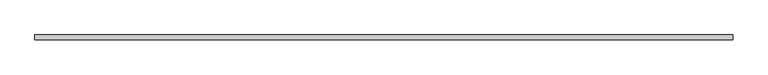
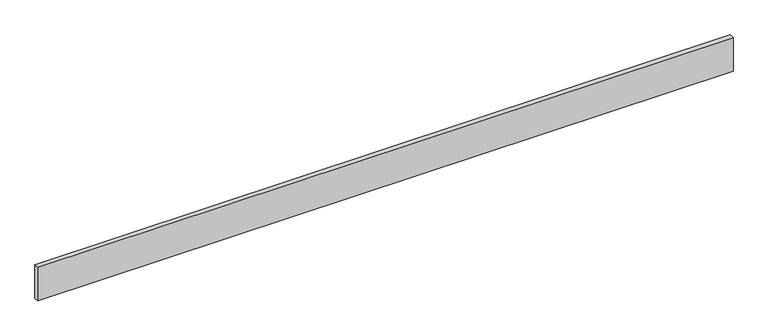
"""IFC4 building model written with IfcOpenShell, lengths in millimetres: proxy geometry, Footer003 : Footer003."""

from ifc_helpers import new_model, si_unit, frame, origin, place, context, project, spatial, polyline, outline, extrude, source, transform, mapped, element, save


def generic_models_1a1cdef9(model_context):
    return source(origin(), model_context, "Body", "SweptSolid", [
        extrude(outline(polyline([(14383.0178845, -4469.7753493), (14383.0178845, -4483.5542972), (12383.0178845, -4483.5542972), (12383.0178845, -4469.7753493), (14383.0178845, -4469.7753493)])), frame((0.0, 0.0, 36582.096), z_axis=(0.0, 0.0, 1.0), x_axis=(1.0, 0.0, 0.0)), (0.0, 0.0, 1.0), 101.6),
    ])


if __name__ == "__main__":
    model = new_model("IFC4")
    model_context = context("Model", 3, world=origin())
    ifc_project = project(units=[si_unit("LENGTHUNIT", "METRE", prefix="MILLI")], contexts=[model_context])
    site = spatial("IfcSite", under=ifc_project)
    building = spatial("IfcBuilding", under=site)
    placement = place(None, origin())
    generic_models_shape = generic_models_1a1cdef9(model_context)
    element("IfcBuildingElementProxy", 1, Name="Footer003 : Footer003", ObjectType="Footer003 : Footer003", at=placement, inside=building, context=model_context, shape_type="MappedRepresentation", body=[
        mapped(generic_models_shape, transform((0.0, 0.0, 0.0), x_axis=(1.0, 0.0, 0.0), y_axis=(0.0, 1.0, 0.0), z_axis=(0.0, 0.0, 1.0))),
    ])
    save(model, "model.ifc")

# Revit data of these elements
# Type "Footer003 : Footer003"
#   NameOverride = "Footer003"
# Element 1 (IfcBuildingElementProxy, "Footer003 : Footer003")
#   Materials on its faces: "FOOTER MATERIAL TBD"
# Materials
#   "FOOTER MATERIAL TBD": class "Unassigned", colour RGB 148 103 60, transparency 0
